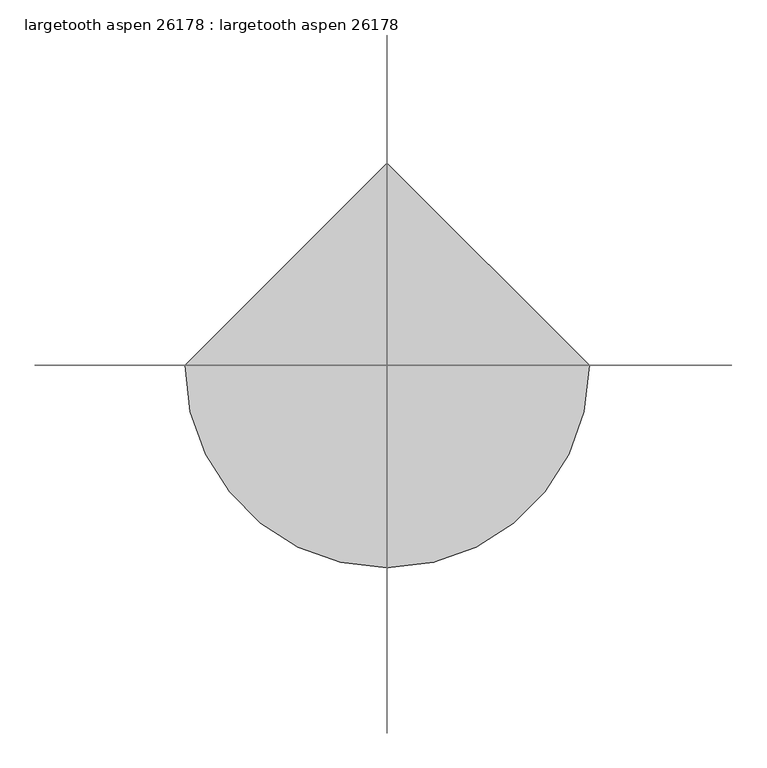
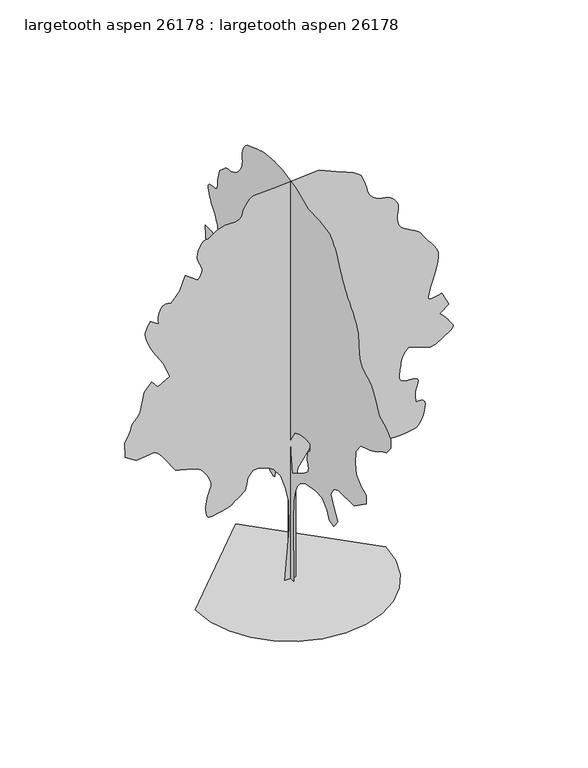
"""IFC4 building model written with IfcOpenShell, lengths in millimetres: proxy geometry, largetooth aspen 26178 : largetooth aspen 26178."""

from ifc_helpers import new_model, si_unit, origin, place, context, project, spatial, triangles, source, transform, mapped, element, save


def largetooth_aspen_26178_largetooth_aspen_26178_f6cd7aa4(model_context):
    return source(origin(), model_context, "Body", "Tessellation", [
        triangles([(93.1061447, 0.000407, 0.0055275), (-104.1894253, 0.000407, 0.0055275), (-22.9504001, 0.0003503, 951.6658939), (-34.5559031, 0.0003185, 1485.5251682), (-92.5836657, 0.0003019, 1764.061219), (-173.8237105, 0.0002874, 2007.7790462), (-301.4849952, 0.000277, 2181.8628971), (-405.9347789, 0.0002735, 2239.8916225), (-568.4133425, 0.0002701, 2297.9204933), (-684.470866, 0.0002701, 2297.9204933), (-765.710166, 0.000277, 2181.8628971), (-800.5284622, 0.000286, 2030.9895481), (-803.4037228, 0.000287, 2013.4305908), (-808.6158319, 0.0002881, 1994.9546837), (-818.4938627, 0.0002893, 1974.6550507), (-835.3797506, 0.0002907, 1951.6121258), (-861.6001705, 0.0002923, 1924.9168076), (-899.4969126, 0.0002942, 1893.6518555), (-951.4017385, 0.0002963, 1856.9058426), (-1000.9367964, 0.0002984, 1821.7851665), (-1035.041328, 0.0003, 1794.7824543), (-1061.0280413, 0.0003013, 1774.0764507), (-1086.2019407, 0.0003023, 1757.8357269), (-1117.8706472, 0.0003031, 1744.2340862), (-1163.3467958, 0.0003038, 1731.4425705), (-1229.9353912, 0.0003046, 1717.6377445), (-1303.2575146, 0.0003056, 1701.9735844), (-1364.6008633, 0.0003064, 1687.5234489), (-1414.7786144, 0.000307, 1678.356712), (-1454.6032185, 0.000307, 1678.5242889), (-1484.8875618, 0.0003062, 1692.0929375), (-1506.439444, 0.0003043, 1723.119096), (-1520.076693, 0.0003012, 1775.66647), (-1526.0305447, 0.0002975, 1838.229221), (-1525.0830734, 0.000294, 1896.7304466), (-1518.8575813, 0.0002907, 1951.3759483), (-1508.9769344, 0.0002877, 2002.3662952), (-1497.0669056, 0.0002848, 2049.9049633), (-1484.7505062, 0.0002822, 2094.1948471), (-1473.6532185, 0.0002797, 2135.4418934), (-1462.0149754, 0.0002776, 2171.5098953), (-1448.7511047, 0.0002758, 2202.2997311), (-1436.5031605, 0.000274, 2231.0600395), (-1427.9079002, 0.0002723, 2261.0397503), (-1425.6065872, 0.0002702, 2295.4845955), (-1432.2385952, 0.0002677, 2337.6435047), (-1450.4427166, 0.0002645, 2390.7649715), (-1477.2752357, 0.0002611, 2448.2171333), (-1507.353923, 0.000258, 2500.7976448), (-1539.6676483, 0.0002552, 2547.8968048), (-1573.1981598, 0.0002527, 2588.9178474), (-1606.9320019, 0.0002507, 2623.2079056), (-1639.8528122, 0.0002491, 2650.2080017), (-1670.950042, 0.0002479, 2669.3088707), (-1706.2051575, 0.000247, 2684.2184258), (-1751.2088058, 0.0002461, 2699.1535606), (-1804.330418, 0.0002453, 2714.0634064), (-1863.9491627, 0.0002444, 2728.9985413), (-1928.439703, 0.0002435, 2743.908387), (-1996.1788822, 0.0002426, 2758.8182327), (-2065.5412182, 0.0002417, 2773.7533676), (-2262.8354256, 0.0002244, 3063.8972855), (-2307.8392193, 0.0002208, 3124.7302002), (-2344.3134464, 0.0002181, 3169.7390808), (-2373.6809853, 0.0002162, 3201.539756), (-2397.3664581, 0.0002149, 3222.7742157), (-2416.7872204, 0.0002141, 3236.1091576), (-2433.3683304, 0.0002137, 3244.1609917), (-2448.5269981, 0.0002133, 3249.5711266), (-2773.4740242, 0.0002154, 3214.7732506), (-2970.7811668, 0.0002078, 3342.4334816), (-2982.3888885, 0.0001919, 3609.3616653), (-2960.1129227, 0.0001895, 3649.1127274), (-2938.5738304, 0.0001872, 3688.6606041), (-2918.4317459, 0.0001848, 3727.8273994), (-2900.4229614, 0.0001825, 3766.3590591), (-2885.2846413, 0.0001803, 3804.0779778), (-2873.6769196, 0.0001781, 3840.78097), (-2866.3363792, 0.000176, 3876.2901398), (-2854.8809738, 0.000174, 3909.843615), (-2833.1131165, 0.0001721, 3941.5934212), (-2804.8174599, 0.0001702, 3972.5051971), (-2773.8803947, 0.0001684, 4003.6457382), (-2744.1877304, 0.0001665, 4035.9798111), (-2719.5499901, 0.0001644, 4070.5745018), (-2703.8526924, 0.0001621, 4108.3951584), (-2634.2060715, 0.0001414, 4456.5779755), (-2494.950618, 0.0001324, 4607.4283607), (-2390.4982727, 0.00014, 4479.7681297), (-2169.9909473, 0.0001331, 4595.8459282), (-2286.0485435, 0.0001158, 4885.9645569), (-2471.7375, 9.85e-05, 5176.1084747), (-2494.0692764, 9.6e-05, 5217.3577011), (-2519.6494011, 9.3e-05, 5268.7673538), (-2546.0425575, 8.96e-05, 5326.2475662), (-2570.8076157, 8.6e-05, 5385.7596313), (-2591.5086777, 8.26e-05, 5443.2398438), (-2605.7325188, 7.95e-05, 5494.6494965), (-2611.0159172, 7.71e-05, 5535.8993042), (-2608.2980598, 7.5e-05, 5570.3669678), (-2600.7287544, 7.3e-05, 5604.2503647), (-2589.0701637, 7.1e-05, 5637.6006546), (-2574.1858978, 6.9e-05, 5670.544574), (-2556.863118, 6.71e-05, 5703.2088593), (-2537.9197975, 6.52e-05, 5735.6446701), (-2518.1611198, 6.32e-05, 5768.0037415), (-2367.2877708, 6.95e-05, 5663.5595352), (-2372.0934368, 6.75e-05, 5695.9697662), (-2375.8831764, 6.56e-05, 5728.8881058), (-2377.6407726, 6.35e-05, 5762.8226624), (-2376.3555313, 6.14e-05, 5798.2809631), (-2371.00891, 5.92e-05, 5835.7711166), (-2360.5873077, 5.68e-05, 5875.8018127), (-2344.077269, 5.42e-05, 5918.8799973), (-2322.4899239, 5.2e-05, 5956.5480469), (-2297.8569798, 5.05e-05, 5981.4145523), (-2270.6865452, 4.97e-05, 5995.6131042), (-2241.4867287, 4.93e-05, 6001.3028732), (-2210.7630226, 4.94e-05, 6000.5918701), (-2179.0257156, 4.97e-05, 5995.6131042), (-2146.7804455, 5.01e-05, 5988.501329), (-1995.9070965, 3.97e-05, 6162.5924469), (-1891.4573673, 2.45e-05, 6417.9129089), (-1670.950042, 3.42e-05, 6255.4298035), (-1648.8215961, 3.24e-05, 6285.3250717), (-1628.2145691, 3.06e-05, 6315.3988174), (-1610.6529957, 2.88e-05, 6345.8789337), (-1597.6609108, 2.69e-05, 6376.9683151), (-1590.7597332, 2.5e-05, 6408.8960175), (-1591.4684109, 2.31e-05, 6441.814357), (-1601.3160656, 2.1e-05, 6475.9523895), (-1617.3536041, 1.89e-05, 6510.877002), (-1634.407069, 1.68e-05, 6546.3864624), (-1650.6477928, 1.46e-05, 6583.140033), (-1664.2495789, 1.23e-05, 6621.7225616), (-1673.3859398, 9.9e-06, 6662.7183151), (-1676.2282082, 7.3e-06, 6706.761557), (-1670.950042, 4.4e-06, 6754.488295), (-1658.2957272, 1.5e-06, 6803.2306686), (-1640.7672913, -1.2e-06, 6848.9505524), (-1619.1798008, -3.6e-06, 6889.9968842), (-1594.3462875, -5.7e-06, 6924.7441818), (-1567.0742603, -7.3e-06, 6951.5663818), (-1538.1767509, -8.4e-06, 6968.8641632), (-1508.471442, -8.7e-06, 6974.9853012), (-1475.2102455, -9.2e-06, 6983.3417679), (-1435.6574272, -1.05e-05, 7004.9067307), (-1390.6206413, -1.23e-05, 7034.3706299), (-1340.9153904, -1.42e-05, 7066.4762283), (-1287.3545609, -1.59e-05, 7095.9401276), (-1230.7481323, -1.72e-05, 7117.504509), (-1171.9065931, -1.77e-05, 7125.861557), (-1111.9499331, -1.77e-05, 7125.5313446), (-1053.2124573, -1.77e-05, 7125.9882935), (-998.3307781, -1.79e-05, 7129.5188919), (-949.9463768, -1.85e-05, 7138.307309), (-910.695793, -1.94e-05, 7154.6138718), (-883.2205805, -2.1e-05, 7180.6744904), (-870.1599678, -2.32e-05, 7218.6983322), (-859.1973375, -2.62e-05, 7267.6691803), (-837.8816328, -2.94e-05, 7321.8984283), (-808.6488241, -3.27e-05, 7376.76194), (-773.9321205, -3.57e-05, 7427.5367477), (-736.1725794, -3.82e-05, 7469.5992966), (-697.8033371, -3.99e-05, 7498.2504547), (-661.2603642, -4.05e-05, 7508.8422501), (-324.6980224, -4.19e-05, 7532.0576935), (510.9103117, -4.54e-05, 7590.0965927), (928.7119898, -3.43e-05, 7404.3974625), (997.9725878, -3.27e-05, 7376.9148376), (1065.003162, -3.1e-05, 7348.7462082), (1127.5632969, -2.92e-05, 7319.1294113), (1183.4279829, -2.73e-05, 7287.4051849), (1230.3570225, -2.53e-05, 7252.8102036), (1266.1201012, -2.3e-05, 7214.6852051), (1288.4873405, -2.05e-05, 7172.2924438), (1303.3743679, -1.8e-05, 7130.6618454), (1318.0580647, -1.58e-05, 7093.7303787), (1332.3378616, -1.37e-05, 7059.0086609), (1346.0081028, -1.16e-05, 7024.0834671), (1358.8656029, -9.4e-06, 6986.5171555), (1370.7070312, -6.9e-06, 6943.8959198), (1381.3319641, -3.9e-06, 6893.7565384), (1397.2017803, -8e-07, 6841.9149353), (1423.0183731, 2e-06, 6795.9665771), (1455.9391834, 4.3e-06, 6756.1137772), (1493.1248497, 6.3e-06, 6722.5350128), (1531.7301968, 7.9e-06, 6695.4843384), (1568.915863, 9.2e-06, 6675.1134888), (1601.8392895, 1e-05, 6661.6259399), (1632.2912098, 1.04e-05, 6653.548526), (1663.5535458, 1.08e-05, 6648.1133926), (1695.0215378, 1.1e-05, 6643.6683151), (1726.0831593, 1.13e-05, 6638.6389709), (1756.1288544, 1.18e-05, 6631.3492996), (1784.5513927, 1.24e-05, 6620.2238159), (1810.7387478, 1.34e-05, 6603.6126205), (1836.0828403, 1.48e-05, 6581.0320221), (1861.4244621, 1.64e-05, 6553.8028702), (1885.3461124, 1.82e-05, 6522.9169647), (1906.4256397, 2.02e-05, 6489.3887787), (1923.2429272, 2.23e-05, 6454.2351105), (1934.3756779, 2.45e-05, 6418.4721771), (1938.4015949, 2.66e-05, 6383.0900345), (1934.8836411, 2.9e-05, 6341.7640686), (1927.3043072, 3.21e-05, 6289.6434128), (1920.1313438, 3.57e-05, 6230.2325043), (1917.8301762, 3.94e-05, 6166.9613663), (1924.8685547, 4.32e-05, 6103.2838577), (1945.7117592, 4.69e-05, 6042.6538376), (1984.8250694, 5.01e-05, 5988.501329), (2039.569693, 5.28e-05, 5943.162236), (2101.6243355, 5.51e-05, 5904.3256531), (2166.9277622, 5.72e-05, 5868.5371399), (2231.4183025, 5.94e-05, 5832.3166763), (2291.0370472, 6.18e-05, 5792.2609818), (2341.7227615, 6.46e-05, 5744.890036), (2379.4162457, 6.81e-05, 5686.7749786), (2417.9887459, 7.19e-05, 5621.9795151), (2469.1466698, 7.58e-05, 5556.3713104), (2525.585376, 7.98e-05, 5489.1376236), (2580.0024033, 8.4e-05, 5419.4657135), (2625.0618622, 8.83e-05, 5346.5422577), (2653.4845459, 9.29e-05, 5269.5800949), (2657.9549126, 9.78e-05, 5187.7164871), (2641.5719009, 0.0001035, 5093.1519104), (2615.0543335, 0.00011, 4983.9574127), (2582.4409172, 0.0001169, 4868.2862755), (2547.7697777, 0.0001237, 4754.2147499), (2515.1639191, 0.0001299, 4649.8972801), (2488.6361778, 0.000135, 4563.4609863), (2472.2607239, 0.0001386, 4502.9835732), (2471.4479828, 0.0001408, 4466.6872421), (2487.0816216, 0.000142, 4445.6050987), (2516.4161682, 0.0001425, 4437.2230522), (2556.710511, 0.0001424, 4438.9758522), (2605.2247009, 0.0001419, 4448.3482452), (2659.2248932, 0.000141, 4462.8008514), (2715.9685226, 0.00014, 4479.7681297), (2843.6287537, 0.0001552, 4224.4476677), (2681.1706467, 0.0001628, 4096.7874367), (2705.9862831, 0.0001642, 4074.3338654), (2730.6243141, 0.0001655, 4051.3466057), (2754.8559746, 0.000167, 4027.3692902), (2778.4777885, 0.0001685, 4001.8420692), (2801.2868614, 0.0001701, 3974.3085754), (2823.0802986, 0.0001719, 3944.2351204), (2843.6287537, 0.0001739, 3911.1135956), (2865.6250854, 0.0001758, 3878.8553902), (2888.8408195, 0.0001775, 3850.6614716), (2908.8050079, 0.000179, 3824.931356), (2921.0478653, 0.0001805, 3799.9886925), (2921.1240234, 0.0001821, 3774.2329971), (2904.5378265, 0.0001837, 3746.0643677), (2866.8441971, 0.0001857, 3713.8064529), (2611.523735, 0.000196, 3539.7150444), (2507.076622, 0.0001967, 3528.1073227), (2124.0931675, 0.0001891, 3655.7675537), (2096.88727, 0.0001908, 3628.2340599), (2070.5983223, 0.0001925, 3599.5829018), (2046.1355713, 0.0001943, 3568.6964149), (2024.4110252, 0.0001964, 3534.4319366), (2006.3439594, 0.0001987, 3495.74767), (1992.8439114, 0.0002013, 3451.4500832), (1984.8250694, 0.0002043, 3400.4470917), (1979.2422707, 0.0002073, 3350.9425552), (1972.8464401, 0.0002097, 3309.9723816), (1966.2475697, 0.0002118, 3274.6916862), (1960.0550697, 0.0002138, 3242.2305862), (1954.8784962, 0.0002157, 3209.7947754), (1951.3250793, 0.0002178, 3174.4887909), (1950.0068459, 0.0002203, 3133.5186172), (1959.0060059, 0.0002226, 3094.8599304), (1982.2191238, 0.0002242, 3067.1485405), (2013.9564308, 0.0002253, 3048.55578), (2048.5358608, 0.000226, 3037.3035599), (2080.2731678, 0.0002263, 3031.5123436), (2103.4861404, 0.0002265, 3029.3787529), (2112.4854458, 0.0002265, 3029.0738297), (2125.1752235, 0.0002264, 3029.9630196), (2157.148708, 0.0002264, 3030.4202591), (2199.274625, 0.0002266, 3027.2451622), (2242.4164684, 0.0002272, 3017.1614754), (2277.4354065, 0.0002284, 2996.942942), (2295.2001652, 0.0002304, 2963.2880196), (2286.5717674, 0.0002334, 2913.021611), (2265.7615551, 0.0002368, 2855.3635025), (2252.261507, 0.0002401, 2801.3633102), (2244.8497501, 0.0002431, 2750.4108971), (2242.3122597, 0.000246, 2701.871418), (2243.429924, 0.0002488, 2655.1864769), (2246.9833408, 0.0002515, 2609.7203568), (2251.7533985, 0.0002541, 2564.8385033), (2291.2047695, 0.0002539, 2569.2835808), (2328.629084, 0.0002538, 2570.4774033), (2361.9894024, 0.0002541, 2565.1434265), (2389.2612843, 0.000255, 2550.1065536), (2408.4128769, 0.0002567, 2522.0472198), (2417.4120369, 0.0002593, 2477.7574814), (2414.2319984, 0.0002631, 2413.9754734), (2401.476091, 0.0002675, 2341.0953289), (2383.2389774, 0.0002716, 2272.8811787), (2359.7236977, 0.0002752, 2211.166777), (2331.1309662, 0.0002784, 2157.7735245), (2297.6690552, 0.000281, 2114.5300884), (2259.536063, 0.0002829, 2083.2677525), (2216.9377911, 0.0002839, 2065.807917), (2176.9759861, 0.0002844, 2057.1795193), (2143.1075592, 0.0002848, 2050.7838341), (2110.049548, 0.0002851, 2046.0136311), (2072.5261116, 0.0002853, 2042.257029), (2025.2567585, 0.0002855, 2038.9092682), (1962.9659386, 0.0002857, 2035.3558514), (1880.3728695, 0.000286, 2030.9895481), (1790.6068371, 0.0002859, 2032.4449825), (1709.3674644, 0.0002851, 2045.4726757), (1635.2326, 0.0002838, 2068.1420769), (1566.7847431, 0.0002819, 2098.5255421), (1502.5989807, 0.0002798, 2134.6977528), (1441.2554867, 0.0002774, 2174.7255421), (1381.3319641, 0.0002749, 2216.6811207), (1126.0062698, 0.0002604, 2460.3989479), (859.0779408, 0.0002535, 2576.4465157), (545.7260645, 0.0002548, 2553.2563614), (394.8527518, 0.0002618, 2437.1885914), (290.4029863, 0.0002708, 2286.3152424), (127.9229058, 0.0002846, 2054.2026661), (93.1061447, 0.0003019, 1764.061219), (93.1061447, 0.0003392, 1137.3575392), (-0.0023708, 90.8437737, 1.11e-05), (-0.0023708, -94.8460457, 0.0), (-0.0023708, -83.2405405, 1160.5629541), (-0.0023708, -94.8460457, 1531.9435558), (-0.0023708, -141.2688208, 1729.2379086), (-0.0023708, -210.9025882, 1880.1112576), (-0.0023708, -303.7481383, 1996.1687084), (-0.0023708, -443.0162001, 2077.4080811), (-0.0023708, -559.0712165, 2100.6185829), (-0.0023708, -791.1838291, 2147.0420574), (-0.0023708, -988.4806526, 2135.4368065), (-0.0023708, -1139.3539289, 1984.5634575), (-0.0023708, -1208.987978, 1845.2955048), (-0.0023708, -1336.648209, 1798.8718849), (-0.0023708, -1475.9163071, 1972.9557358), (-0.0023708, -1325.0429581, 2205.0707829), (-0.0023708, -1255.4089817, 2367.5493828), (-0.0023708, -1336.648209, 2506.8150101), (-0.0023708, -1487.521558, 2576.4465157), (-0.0023708, -1974.9572124, 2576.4465157), (-0.0023708, -2357.9431377, 2843.3746994), (-0.0023708, -2357.9431377, 3005.8583862), (-0.0023708, -2195.4645378, 3075.479718), (-0.0023708, -2044.5913342, 3214.7476707), (-0.0023708, -2009.7755814, 3412.0548134), (-0.0023708, -2032.9860832, 3644.159832), (-0.0023708, -2183.8592869, 3841.466684), (-0.0023708, -2450.787616, 3934.3037498), (-0.0023708, -2495.4866318, 3951.778846), (-0.0023708, -2539.7763702, 3969.5332855), (-0.0023708, -2583.2536583, 3987.8975716), (-0.0023708, -2625.5191017, 4007.2016258), (-0.0023708, -2666.159063, 4027.6995026), (-0.0023708, -2704.7671715, 4049.7211235), (-0.0023708, -2740.9367661, 4073.5717026), (-0.0023708, -2775.734642, 4097.0920692), (-0.0023708, -2810.5580978, 4118.1742126), (-0.0023708, -2845.381263, 4137.223922), (-0.0023708, -2880.2047188, 4154.6484398), (-0.0023708, -2915.0025948, 4170.8535553), (-0.0023708, -2949.8260506, 4186.2459297), (-0.0023708, -2984.6495064, 4201.2319336), (-0.0023708, -3112.3097374, 4363.7156204), (-0.0023708, -3112.3097374, 4526.1993073), (-0.0023708, -2961.4337723, 4665.46726), (-0.0023708, -2764.1522095, 4769.9120476), (-0.0023708, -2636.4666893, 5013.6247879), (-0.0023708, -2508.8189575, 5199.3239182), (-0.0023708, -2230.2829067, 5350.1995926), (-0.0023708, -2149.0435341, 5477.860405), (-0.0023708, -2125.8305614, 5733.180867), (-0.0023708, -2102.6200596, 5942.0698608), (-0.0023708, -2077.7179459, 5994.1655182), (-0.0023708, -2052.6126469, 6045.3211166), (-0.0023708, -2027.0983612, 6094.647757), (-0.0023708, -2000.9769905, 6141.2315414), (-0.0023708, -1974.0453495, 6184.1824081), (-0.0023708, -1946.0953114, 6222.5364624), (-0.0023708, -1916.9309578, 6255.4298035), (-0.0023708, -1880.7588924, 6294.3169647), (-0.0023708, -1835.0490372, 6347.6061539), (-0.0023708, -1784.4624447, 6409.8360764), (-0.0023708, -1733.6777538, 6475.4948593), (-0.0023708, -1687.355872, 6539.1473694), (-0.0023708, -1650.170351, 6595.2811523), (-0.0023708, -1626.7896561, 6638.4104965), (-0.0023708, -1609.9062389, 6674.6559586), (-0.0023708, -1589.7741829, 6713.7465958), (-0.0023708, -1567.4070889, 6755.6568283), (-0.0023708, -1543.8256794, 6800.4366531), (-0.0023708, -1520.0386139, 6848.0360733), (-0.0023708, -1497.0642895, 6898.4806686), (-0.0023708, -1475.9163071, 6951.7698578), (-0.0023708, -1452.6372047, 7005.1352051), (-0.0023708, -1423.2671951, 7056.0623291), (-0.0023708, -1388.8223499, 7104.957019), (-0.0023708, -1350.3185955, 7152.2262268), (-0.0023708, -1308.7667713, 7198.2763229), (-0.0023708, -1265.188036, 7243.513678), (-0.0023708, -1220.5932289, 7288.3446625), (-0.0023708, -895.6335583, 7346.3585632), (-0.0023708, -547.4659656, 7357.9659943), (-0.0023708, -176.0855819, 7520.4496811), (-0.0023708, 264.9268161, 7613.2870377), (-0.0023708, 324.5456334, 7615.7252609), (-0.0023708, 383.7580439, 7617.8588516), (-0.0023708, 442.1602203, 7619.3825958), (-0.0023708, 499.3406327, 7619.9924423), (-0.0023708, 554.9005408, 7619.3825958), (-0.0023708, 608.4284509, 7617.2490051), (-0.0023708, 659.5204994, 7613.2870377), (-0.0023708, 708.649114, 7608.2065338), (-0.0023708, 756.9649876, 7602.5423447), (-0.0023708, 805.0801466, 7595.6340454), (-0.0023708, 853.6016762, 7586.8962067), (-0.0023708, 903.136734, 7575.7457245), (-0.0023708, 954.2948032, 7561.5215927), (-0.0023708, 1007.6881285, 7543.6657059), (-0.0023708, 1344.2529774, 7427.6129059), (-0.0023708, 1373.9607571, 7402.5429245), (-0.0023708, 1402.8557957, 7376.228833), (-0.0023708, 1430.1278229, 7347.5015167), (-0.0023708, 1454.9613361, 7315.141864), (-0.0023708, 1476.5488266, 7277.8801849), (-0.0023708, 1494.0772625, 7234.5479462), (-0.0023708, 1506.7315773, 7183.8748764), (-0.0023708, 1511.0952644, 7135.4627151), (-0.0023708, 1507.5418476, 7096.3970764), (-0.0023708, 1500.9454479, 7061.7770966), (-0.0023708, 1496.1727741, 7026.7507462), (-0.0023708, 1498.1031796, 6986.4659958), (-0.0023708, 1511.6032276, 6935.996402), (-0.0023708, 1541.5473301, 6870.5405136), (-0.0023708, 1582.5555828, 6804.0434097), (-0.0023708, 1625.189463, 6752.1768082), (-0.0023708, 1668.2270977, 6712.4769058), (-0.0023708, 1710.4546074, 6682.5298965), (-0.0023708, 1750.6525898, 6659.8987198), (-0.0023708, 1787.5994625, 6642.1439896), (-0.0023708, 1820.0833809, 6626.8024841), (-0.0023708, 1849.9258907, 6615.6775818), (-0.0023708, 1879.7682552, 6610.2418671), (-0.0023708, 1909.6107651, 6607.6257477), (-0.0023708, 1939.4557457, 6605.0346268), (-0.0023708, 1969.2981102, 6599.5739136), (-0.0023708, 1999.14062, 6588.4484299), (-0.0023708, 2028.9829845, 6568.7891647), (-0.0023708, 2203.0693062, 6417.9129089), (-0.0023708, 2272.7008118, 6197.4159027), (-0.0023708, 2270.435107, 6162.7197647), (-0.0023708, 2269.4877811, 6128.8613663), (-0.0023708, 2271.179393, 6096.6034515), (-0.0023708, 2276.8307922, 6066.8093399), (-0.0023708, 2287.7578869, 6040.2411942), (-0.0023708, 2305.2864681, 6017.7367538), (-0.0023708, 2330.7295372, 6000.1087601), (-0.0023708, 2366.121999, 5990.0250732), (-0.0023708, 2409.2282341, 5986.2404205), (-0.0023708, 2454.9736977, 5983.6754608), (-0.0023708, 2498.2855888, 5977.2491089), (-0.0023708, 2534.0819504, 5961.8820236), (-0.0023708, 2557.2947777, 5932.4942825), (-0.0023708, 2562.8319397, 5884.0565414), (-0.0023708, 2554.1452606, 5827.7448624), (-0.0023708, 2538.7528862, 5777.5287415), (-0.0023708, 2517.7724808, 5732.3931244), (-0.0023708, 2492.3292664, 5691.3217941), (-0.0023708, 2463.5359657, 5653.2979523), (-0.0023708, 2432.5073364, 5617.3059631), (-0.0023708, 2400.3636589, 5582.3046112), (-0.0023708, 2375.59613, 5540.0391678), (-0.0023708, 2351.4381569, 5497.9004608), (-0.0023708, 2328.49697, 5455.9402313), (-0.0023708, 2307.3844505, 5414.284053), (-0.0023708, 2288.7053581, 5373.0342453), (-0.0023708, 2273.0741901, 5332.2931274), (-0.0023708, 2261.0955608, 5292.1606934), (-0.0023708, 2254.8700687, 5254.4164856), (-0.0023708, 2255.3450397, 5220.3046143), (-0.0023708, 2261.4003387, 5189.2402313), (-0.0023708, 2271.9235336, 5160.614653), (-0.0023708, 2285.7971054, 5133.8174515), (-0.0023708, 2301.9032444, 5108.2399429), (-0.0023708, 2319.1244316, 5083.2716995), (-0.0023708, 2469.9977806, 5106.4871429), (-0.0023708, 2655.6942947, 5106.4871429), (-0.0023708, 2632.4788513, 4769.9120476), (-0.0023708, 2423.5741608, 4410.1467979), (-0.0023708, 2416.0988903, 4367.9066437), (-0.0023708, 2408.5195564, 4325.9967018), (-0.0023708, 2400.7370373, 4284.6710266), (-0.0023708, 2392.6495949, 4244.2848289), (-0.0023708, 2384.1559273, 4205.0927444), (-0.0023708, 2375.1567673, 4167.4246948), (-0.0023708, 2365.5479061, 4131.6106018), (-0.0023708, 2351.1663712, 4092.901046), (-0.0023708, 2330.0869892, 4047.8924561), (-0.0023708, 2305.5556377, 3998.8448685), (-0.0023708, 2280.8237171, 3947.9433243), (-0.0023708, 2259.134634, 3897.4737305), (-0.0023708, 2243.7397888, 3849.620256), (-0.0023708, 2237.885059, 3806.6435188), (-0.0023708, 2242.6221245, 3768.5435188), (-0.0023708, 2255.8859951, 3733.4915886), (-0.0023708, 2276.2542286, 3700.9796196), (-0.0023708, 2302.3069988, 3670.4995033), (-0.0023708, 2332.6244797, 3641.5181328), (-0.0023708, 2365.7840836, 3613.5782684), (-0.0023708, 2400.3636589, 3586.1462219), (-0.0023708, 2713.7079048, 3655.7675537), (-0.0023708, 2731.0053955, 3606.110701), (-0.0023708, 2747.5915924, 3556.834639), (-0.0023708, 2762.7552017, 3508.3968979), (-0.0023708, 2775.7599312, 3461.1529793), (-0.0023708, 2785.945356, 3415.5345428), (-0.0023708, 2792.5748932, 3371.9482498), (-0.0023708, 2794.9625381, 3330.8257599), (-0.0023708, 2781.5002785, 3291.6333847), (-0.0023708, 2746.9055878, 3253.2540413), (-0.0023708, 2699.9410126, 3215.103463), (-0.0023708, 2649.3188118, 3176.5209343), (-0.0023708, 2603.7768242, 3136.9477684), (-0.0023708, 2572.0523071, 3095.7235405), (-0.0023708, 2562.8319397, 3052.2895638), (-0.0023708, 2571.1886971, 3010.557518), (-0.0023708, 2585.6413033, 2974.3117653), (-0.0023708, 2605.1738319, 2942.6631157), (-0.0023708, 2628.7450676, 2914.6470932), (-0.0023708, 2655.3896622, 2889.3742172), (-0.0023708, 2684.0408203, 2865.9044289), (-0.0023708, 2713.7079048, 2843.3746994), (-0.0023708, 2783.3545258, 2611.2696808), (-0.0023708, 2716.5272095, 2608.9584846), (-0.0023708, 2651.6302986, 2607.7899513), (-0.0023708, 2590.5941986, 2608.8314575), (-0.0023708, 2535.3339088, 2613.225666), (-0.0023708, 2487.7955315, 2622.0902412), (-0.0023708, 2449.8987167, 2636.5428474), (-0.0023708, 2423.5741608, 2657.7008583), (-0.0023708, 2398.2655312, 2683.9137932), (-0.0023708, 2363.2136009, 2712.5649513), (-0.0023708, 2320.0387653, 2743.2479622), (-0.0023708, 2270.3665066, 2775.5823257), (-0.0023708, 2215.8225975, 2809.1102211), (-0.0023708, 2158.0326656, 2843.4508575), (-0.0023708, 2098.6169609, 2878.1981552), (-0.0023708, 2096.1482162, 2840.8347382), (-0.0023708, 2093.7783028, 2803.1919777), (-0.0023708, 2091.6141907, 2764.9143723), (-0.0023708, 2089.7523857, 2725.7219971), (-0.0023708, 2088.2969513, 2685.3360901), (-0.0023708, 2087.3496254, 2643.4008591), (-0.0023708, 2087.01171, 2599.6619591), (-0.0023708, 2085.4216908, 2554.0943916), (-0.0023708, 2079.9734768, 2509.3195084), (-0.0023708, 2069.6534672, 2469.0222588), (-0.0023708, 2053.4457355, 2436.8431183), (-0.0023708, 2030.3368263, 2416.4418926), (-0.0023708, 1999.3108131, 2411.4660336), (-0.0023708, 1959.3490082, 2425.5756374), (-0.0023708, 1914.2462379, 2451.7986008), (-0.0023708, 1868.5363827, 2480.4573166), (-0.0023708, 1822.3160934, 2511.1455597), (-0.0023708, 1775.6894337, 2543.4517273), (-0.0023708, 1728.7603214, 2576.9799133), (-0.0023708, 1681.6281693, 2611.3461296), (-0.0023708, 1634.3918083, 2646.0931366), (-0.0023708, 1355.8582283, 2727.3221901), (-0.0023708, 1077.3221775, 2634.4854149), (-0.0023708, 903.2383266, 2425.5756374), (-0.0023708, 925.671623, 2395.8678577), (-0.0023708, 948.4096247, 2366.9728191), (-0.0023708, 971.754784, 2339.7009373), (-0.0023708, 996.0142771, 2314.8672787), (-0.0023708, 1021.4930271, 2293.2799335), (-0.0023708, 1048.4931959, 2275.7513523), (-0.0023708, 1077.3221775, 2263.0970375), (-0.0023708, 1104.7973173, 2250.7806381), (-0.0023708, 1128.0078192, 2234.2021442), (-0.0023708, 1147.667375, 2214.0700882), (-0.0023708, 1164.4821917, 2191.0957638), (-0.0023708, 1179.1684319, 2165.9904648), (-0.0023708, 1192.4323025, 2139.4627235), (-0.0023708, 1204.984952, 2112.2238338), (-0.0023708, 1172.5694887, 2104.7129551), (-0.0023708, 1139.6486057, 2096.8974438), (-0.0023708, 1105.7091803, 2088.4722313), (-0.0023708, 1070.2508068, 2079.1326851), (-0.0023708, 1032.7604353, 2068.576498), (-0.0023708, 992.7325733, 2056.4962761), (-0.0023708, 949.6593304, 2042.5897121), (-0.0023708, 906.5885582, 2025.6403107), (-0.0023708, 866.5607689, 2005.0332836), (-0.0023708, 829.0703974, 1981.383419), (-0.0023708, 793.6094805, 1955.2951859), (-0.0023708, 759.6725985, 1927.3806107), (-0.0023708, 726.7517155, 1898.2467785), (-0.0023708, 694.3362522, 1868.5060066), (-0.0023708, 694.3362522, 1706.0274067), (-0.0023708, 652.3120005, 1679.1287579), (-0.0023708, 611.8117109, 1654.968314), (-0.0023708, 574.3543679, 1636.2916924), (-0.0023708, 541.4665134, 1625.8370979), (-0.0023708, 514.6695299, 1626.3450611), (-0.0023708, 495.4849088, 1640.556403), (-0.0023708, 485.4341414, 1671.2116539), (-0.0023708, 480.5294263, 1705.9588062), (-0.0023708, 476.0285382, 1733.1976959), (-0.0023708, 472.3404639, 1756.7815762), (-0.0023708, 469.8715739, 1780.5661709), (-0.0023708, 469.025768, 1808.4147617), (-0.0023708, 470.2094167, 1844.1778404), (-0.0023708, 473.8288905, 1891.7165085), (-0.0023708, 476.7727515, 1943.7229271), (-0.0023708, 476.0615667, 1990.8550793), (-0.0023708, 472.3074354, 2033.9283222), (-0.0023708, 466.1149355, 2073.7529263), (-0.0023708, 458.0961662, 2111.1417778), (-0.0023708, 448.8581763, 2146.9074726), (-0.0023708, 439.0131741, 2181.8578102), (-0.0023708, 241.7168229, 2193.4630611), (-0.0023708, 137.2665396, 1996.1687084), (-0.0023708, 79.2382684, 1659.6039322), (-0.0023708, 79.2382684, 1230.1970032), (-0.0023708, 79.2382684, 591.8879997), (-0.0022508, -48.4240337, 2030.9844612), (-0.0022508, -2.0012081, 2402.3651356), (-0.0022508, 9.6043397, 2622.8776932), (-0.0022508, -129.6633155, 2843.3746994), (-0.0022508, -280.5376365, 2913.021611), (-0.0022508, -454.621451, 2936.2117653), (-0.0022508, -617.0999783, 2936.2117653), (-0.0022508, -617.0999783, 2796.9691017), (-0.0022508, -535.8607146, 2727.3221901), (-0.0022508, -512.6502128, 2564.8385033), (-0.0022508, -522.5282799, 2554.7295273), (-0.0022508, -532.0024836, 2543.6043343), (-0.0022508, -540.6638735, 2530.4344986), (-0.0022508, -548.1085862, 2514.226767), (-0.0022508, -553.9277441, 2493.9573647), (-0.0022508, -557.717411, 2468.6158882), (-0.0022508, -559.0712165, 2437.1808884), (-0.0022508, -555.6879564, 2404.7324329), (-0.0022508, -546.2137527, 2376.5486881), (-0.0022508, -531.6646408, 2351.915744), (-0.0022508, -513.0540762, 2330.1250683), (-0.0022508, -491.4006014, 2310.4679832), (-0.0022508, -467.7151285, 2292.2308697), (-0.0022508, -443.0162001, 2274.7022884), (-1711.8591728, 0.0, 0.0031267), (-1666.6040863, -392.2441901, 0.0031033), (-1537.7144245, -752.4590126, 0.0030819), (-1335.5154293, -1070.3218781, 0.0030629), (-1070.3218781, -1335.5154293, 0.0030471), (-752.4590126, -1537.7144245, 0.0030351), (-392.2441901, -1666.6040863, 0.0030274), (7.5e-05, -1711.8591728, 0.0030247), (392.2441901, -1666.6040863, 0.0030274), (752.4590126, -1537.7144245, 0.0030351), (1070.3218781, -1335.5154293, 0.0030471), (1335.5154293, -1070.3218781, 0.0030629), (1537.7144245, -752.4590126, 0.0030819), (1666.6040863, -392.2441901, 0.0031033), (1711.8591728, 0.0001497, 0.0031267), (-0.0002251, 1711.8591728, 0.0032287)], [[122, 123, 124], [87, 88, 89], [1, 2, 3], [329, 1, 3], [329, 3, 4], [328, 329, 4], [328, 4, 5], [105, 106, 107], [327, 328, 5], [327, 5, 6], [104, 105, 107], [238, 239, 240], [238, 240, 241], [237, 238, 241], [236, 237, 241], [103, 104, 107], [86, 87, 89], [235, 236, 241], [102, 103, 107], [101, 102, 107], [100, 101, 107], [99, 100, 107], [98, 99, 107], [97, 98, 107], [96, 97, 107], [327, 6, 7], [326, 327, 7], [95, 96, 107], [70, 71, 72], [69, 70, 72], [69, 72, 73], [69, 73, 74], [69, 74, 75], [69, 75, 76], [69, 76, 77], [69, 77, 78], [94, 95, 107], [234, 235, 241], [93, 94, 107], [69, 78, 79], [69, 79, 80], [69, 80, 81], [69, 81, 82], [69, 82, 83], [69, 83, 84], [69, 84, 85], [68, 69, 85], [325, 326, 7], [325, 7, 8], [67, 68, 85], [92, 93, 107], [91, 92, 107], [60, 61, 62], [67, 85, 86], [67, 86, 89], [67, 89, 90], [66, 67, 90], [65, 66, 90], [64, 65, 90], [63, 64, 90], [62, 63, 90], [60, 62, 90], [59, 60, 90], [58, 59, 90], [57, 58, 90], [56, 57, 90], [55, 56, 90], [54, 55, 90], [53, 54, 90], [284, 285, 286], [283, 284, 286], [282, 283, 286], [282, 286, 287], [281, 282, 287], [280, 281, 287], [279, 280, 287], [279, 287, 288], [278, 279, 288], [277, 278, 288], [277, 288, 289], [276, 277, 289], [275, 276, 289], [275, 289, 290], [52, 53, 90], [325, 8, 9], [121, 122, 124], [275, 290, 291], [30, 31, 32], [29, 30, 32], [29, 32, 33], [28, 29, 33], [28, 33, 34], [27, 28, 34], [27, 34, 35], [27, 35, 36], [26, 27, 36], [26, 36, 37], [26, 37, 38], [25, 26, 38], [25, 38, 39], [24, 25, 39], [23, 24, 39], [22, 23, 39], [21, 22, 39], [20, 21, 39], [20, 39, 40], [20, 40, 41], [20, 41, 42], [19, 20, 42], [19, 42, 43], [18, 19, 43], [18, 43, 44], [17, 18, 44], [16, 17, 44], [15, 16, 44], [14, 15, 44], [13, 14, 44], [12, 13, 44], [11, 12, 44], [11, 44, 45], [11, 45, 46], [10, 11, 46], [10, 46, 47], [10, 47, 48], [10, 48, 49], [10, 49, 50], [10, 50, 51], [252, 253, 254], [251, 252, 254], [251, 254, 255], [250, 251, 255], [249, 250, 255], [249, 255, 256], [248, 249, 256], [247, 248, 256], [246, 247, 256], [245, 246, 256], [245, 256, 257], [245, 257, 258], [244, 245, 258], [243, 244, 258], [242, 243, 258], [241, 242, 258], [234, 241, 258], [233, 234, 258], [274, 275, 291], [324, 325, 9], [51, 52, 90], [10, 51, 90], [9, 10, 90], [324, 9, 90], [323, 324, 90], [323, 90, 91], [323, 91, 107], [323, 107, 108], [323, 108, 109], [323, 109, 110], [323, 110, 111], [323, 111, 112], [323, 112, 113], [323, 113, 114], [323, 114, 115], [323, 115, 116], [323, 116, 117], [323, 117, 118], [323, 118, 119], [323, 119, 120], [323, 120, 121], [323, 121, 124], [323, 124, 125], [323, 125, 126], [323, 126, 127], [323, 127, 128], [323, 128, 129], [322, 323, 129], [322, 129, 130], [167, 168, 169], [274, 291, 292], [296, 297, 298], [296, 298, 299], [295, 296, 299], [294, 295, 299], [294, 299, 300], [293, 294, 300], [293, 300, 301], [293, 301, 302], [293, 302, 303], [293, 303, 304], [293, 304, 305], [293, 305, 306], [293, 306, 307], [293, 307, 308], [293, 308, 309], [293, 309, 310], [293, 310, 311], [293, 311, 312], [293, 312, 313], [293, 313, 314], [293, 314, 315], [293, 315, 316], [293, 316, 317], [293, 317, 318], [293, 318, 319], [292, 293, 319], [274, 292, 319], [274, 319, 320], [274, 320, 321], [274, 321, 322], [273, 274, 322], [273, 322, 130], [272, 273, 130], [271, 272, 130], [270, 271, 130], [269, 270, 130], [268, 269, 130], [267, 268, 130], [266, 267, 130], [265, 266, 130], [264, 265, 130], [263, 264, 130], [262, 263, 130], [261, 262, 130], [260, 261, 130], [259, 260, 130], [258, 259, 130], [233, 258, 130], [232, 233, 130], [231, 232, 130], [230, 231, 130], [229, 230, 130], [228, 229, 130], [227, 228, 130], [226, 227, 130], [225, 226, 130], [224, 225, 130], [223, 224, 130], [222, 223, 130], [221, 222, 130], [220, 221, 130], [219, 220, 130], [218, 219, 130], [217, 218, 130], [216, 217, 130], [215, 216, 130], [214, 215, 130], [213, 214, 130], [212, 213, 130], [211, 212, 130], [210, 211, 130], [209, 210, 130], [208, 209, 130], [207, 208, 130], [206, 207, 130], [205, 206, 130], [204, 205, 130], [203, 204, 130], [202, 203, 130], [201, 202, 130], [200, 201, 130], [199, 200, 130], [198, 199, 130], [197, 198, 130], [196, 197, 130], [195, 196, 130], [194, 195, 130], [193, 194, 130], [192, 193, 130], [191, 192, 130], [190, 191, 130], [189, 190, 130], [188, 189, 130], [187, 188, 130], [186, 187, 130], [185, 186, 130], [184, 185, 130], [183, 184, 130], [182, 183, 130], [181, 182, 130], [180, 181, 130], [179, 180, 130], [178, 179, 130], [177, 178, 130], [176, 177, 130], [175, 176, 130], [174, 175, 130], [173, 174, 130], [172, 173, 130], [171, 172, 130], [170, 171, 130], [169, 170, 130], [167, 169, 130], [167, 130, 131], [167, 131, 132], [167, 132, 133], [167, 133, 134], [167, 134, 135], [167, 135, 136], [164, 165, 166], [164, 166, 167], [163, 164, 167], [162, 163, 167], [161, 162, 167], [160, 161, 167], [159, 160, 167], [158, 159, 167], [143, 144, 145], [142, 143, 145], [141, 142, 145], [140, 141, 145], [140, 145, 146], [139, 140, 146], [138, 139, 146], [137, 138, 146], [136, 137, 146], [136, 146, 147], [136, 147, 148], [136, 148, 149], [136, 149, 150], [136, 150, 151], [136, 151, 152], [136, 152, 153], [136, 153, 154], [136, 154, 155], [136, 155, 156], [157, 158, 167], [157, 167, 136], [157, 136, 156], [634, 330, 635], [633, 634, 635], [632, 633, 635], [631, 632, 635], [540, 541, 542], [592, 593, 594], [494, 495, 496], [635, 330, 331], [635, 331, 332], [635, 332, 333], [635, 333, 334], [635, 334, 335], [658, 635, 335], [658, 335, 336], [658, 336, 337], [658, 337, 338], [540, 542, 543], [657, 658, 338], [631, 635, 636], [630, 631, 636], [518, 519, 520], [656, 657, 338], [656, 338, 339], [655, 656, 339], [654, 655, 339], [653, 654, 339], [540, 543, 544], [539, 540, 544], [518, 520, 521], [539, 544, 545], [538, 539, 545], [538, 545, 546], [538, 546, 547], [538, 547, 548], [537, 538, 548], [537, 548, 549], [536, 537, 549], [536, 549, 550], [536, 550, 551], [535, 536, 551], [535, 551, 552], [534, 535, 552], [493, 494, 496], [493, 496, 497], [343, 344, 345], [342, 343, 345], [341, 342, 345], [340, 341, 345], [340, 345, 346], [534, 552, 553], [533, 534, 553], [518, 521, 522], [350, 351, 352], [349, 350, 352], [349, 352, 353], [348, 349, 353], [533, 553, 554], [652, 653, 339], [518, 522, 523], [518, 523, 524], [533, 554, 555], [532, 533, 555], [518, 524, 525], [518, 525, 526], [518, 526, 527], [518, 527, 528], [518, 528, 529], [518, 529, 530], [518, 530, 531], [518, 531, 532], [518, 532, 555], [517, 518, 555], [516, 517, 555], [515, 516, 555], [607, 608, 609], [591, 592, 594], [591, 594, 595], [590, 591, 595], [590, 595, 596], [589, 590, 596], [588, 589, 596], [588, 596, 597], [587, 588, 597], [586, 587, 597], [586, 597, 598], [585, 586, 598], [585, 598, 599], [584, 585, 599], [584, 599, 600], [583, 584, 600], [583, 600, 601], [582, 583, 601], [514, 515, 555], [643, 644, 645], [630, 636, 637], [629, 630, 637], [581, 582, 601], [581, 601, 602], [348, 353, 354], [580, 581, 602], [580, 602, 603], [579, 580, 603], [651, 652, 339], [651, 339, 340], [651, 340, 346], [650, 651, 346], [649, 650, 346], [649, 346, 347], [648, 649, 347], [647, 648, 347], [646, 647, 347], [372, 373, 374], [371, 372, 374], [370, 371, 374], [369, 370, 374], [369, 374, 375], [368, 369, 375], [367, 368, 375], [366, 367, 375], [365, 366, 375], [364, 365, 375], [363, 364, 375], [362, 363, 375], [361, 362, 375], [360, 361, 375], [359, 360, 375], [358, 359, 375], [357, 358, 375], [356, 357, 375], [356, 375, 376], [356, 376, 377], [356, 377, 378], [645, 646, 347], [643, 645, 347], [642, 643, 347], [641, 642, 347], [641, 347, 348], [641, 348, 354], [641, 354, 355], [607, 609, 610], [513, 514, 555], [579, 603, 604], [607, 610, 611], [607, 611, 612], [607, 612, 613], [607, 613, 614], [607, 614, 615], [607, 615, 616], [607, 616, 617], [607, 617, 618], [607, 618, 619], [607, 619, 620], [607, 620, 621], [607, 621, 622], [607, 622, 623], [607, 623, 624], [606, 607, 624], [606, 624, 625], [605, 606, 625], [605, 625, 626], [604, 605, 626], [579, 604, 626], [579, 626, 627], [579, 627, 628], [579, 628, 629], [579, 629, 637], [578, 579, 637], [578, 637, 638], [355, 356, 378], [641, 355, 378], [641, 378, 379], [640, 641, 379], [639, 640, 379], [639, 379, 380], [639, 380, 381], [639, 381, 382], [639, 382, 383], [639, 383, 384], [639, 384, 385], [639, 385, 386], [639, 386, 387], [639, 387, 388], [639, 388, 389], [639, 389, 390], [639, 390, 391], [639, 391, 392], [639, 392, 393], [639, 393, 394], [639, 394, 395], [638, 639, 395], [578, 638, 395], [577, 578, 395], [577, 395, 396], [577, 396, 397], [577, 397, 398], [577, 398, 399], [577, 399, 400], [577, 400, 401], [577, 401, 402], [577, 402, 403], [577, 403, 404], [577, 404, 405], [577, 405, 406], [577, 406, 407], [577, 407, 408], [577, 408, 409], [577, 409, 410], [577, 410, 411], [577, 411, 412], [577, 412, 413], [577, 413, 414], [577, 414, 415], [577, 415, 416], [577, 416, 417], [577, 417, 418], [577, 418, 419], [577, 419, 420], [577, 420, 421], [577, 421, 422], [577, 422, 423], [577, 423, 424], [577, 424, 425], [577, 425, 426], [577, 426, 427], [577, 427, 428], [577, 428, 429], [577, 429, 430], [577, 430, 431], [577, 431, 432], [577, 432, 433], [577, 433, 434], [566, 567, 568], [566, 568, 569], [565, 566, 569], [564, 565, 569], [564, 569, 570], [563, 564, 570], [563, 570, 571], [562, 563, 571], [562, 571, 572], [561, 562, 572], [560, 561, 572], [560, 572, 573], [559, 560, 573], [559, 573, 574], [558, 559, 574], [558, 574, 575], [557, 558, 575], [556, 557, 575], [556, 575, 576], [555, 556, 576], [513, 555, 576], [513, 576, 577], [512, 513, 577], [511, 512, 577], [470, 471, 472], [469, 470, 472], [468, 469, 472], [468, 472, 473], [467, 468, 473], [467, 473, 474], [467, 474, 475], [466, 467, 475], [466, 475, 476], [466, 476, 477], [465, 466, 477], [465, 477, 478], [465, 478, 479], [464, 465, 479], [464, 479, 480], [464, 480, 481], [464, 481, 482], [463, 464, 482], [456, 457, 458], [456, 458, 459], [456, 459, 460], [510, 511, 577], [463, 482, 483], [455, 456, 460], [454, 455, 460], [453, 454, 460], [452, 453, 460], [451, 452, 460], [450, 451, 460], [450, 460, 461], [449, 450, 461], [449, 461, 462], [463, 483, 484], [492, 493, 497], [448, 449, 462], [447, 448, 462], [491, 492, 497], [462, 463, 484], [447, 462, 484], [447, 484, 485], [446, 447, 485], [446, 485, 486], [445, 446, 486], [445, 486, 487], [444, 445, 487], [444, 487, 488], [491, 497, 498], [509, 510, 577], [491, 498, 499], [491, 499, 500], [490, 491, 500], [490, 500, 501], [490, 501, 502], [490, 502, 503], [490, 503, 504], [490, 504, 505], [490, 505, 506], [490, 506, 507], [490, 507, 508], [490, 508, 509], [490, 509, 577], [489, 490, 577], [488, 489, 577], [444, 488, 577], [443, 444, 577], [442, 443, 577], [441, 442, 577], [440, 441, 577], [435, 436, 437], [434, 435, 437], [434, 437, 438], [434, 438, 439], [577, 434, 439], [440, 577, 439], [673, 674, 659], [672, 673, 659], [672, 659, 660], [671, 672, 660], [671, 660, 661], [671, 661, 662], [670, 671, 662], [669, 670, 662], [669, 662, 663], [669, 663, 664], [669, 664, 665], [669, 665, 666], [669, 666, 667], [669, 667, 668]], closed=False),
    ])


if __name__ == "__main__":
    model = new_model("IFC4")
    model_context = context("Model", 3, world=origin())
    ifc_project = project(units=[si_unit("LENGTHUNIT", "METRE", prefix="MILLI")], contexts=[model_context])
    site = spatial("IfcSite", under=ifc_project)
    building = spatial("IfcBuilding", under=site)
    placement = place(None, origin())
    largetooth_aspen_26178_largetooth_aspen_26178_shape = largetooth_aspen_26178_largetooth_aspen_26178_f6cd7aa4(model_context)
    element("IfcBuildingElementProxy", 1, Name="largetooth aspen 26178 : largetooth aspen 26178", ObjectType="largetooth aspen 26178 : largetooth aspen 26178", at=placement, inside=building, context=model_context, shape_type="MappedRepresentation", body=[
        mapped(largetooth_aspen_26178_largetooth_aspen_26178_shape, transform((0.0, 0.0, 0.0), x_axis=(1.0, 0.0, 0.0), y_axis=(0.0, 1.0, 0.0), z_axis=(0.0, 0.0, 1.0))),
    ])
    save(model, "model.ifc")

# Revit data of these elements
# Type "largetooth aspen 26178 : largetooth aspen 26178"
#   built-in parameter 1005195 = "RPC-16-G0VG-J3PX-MQ0P-J000-ST1L-LVER-AU"
#   Height = 0
